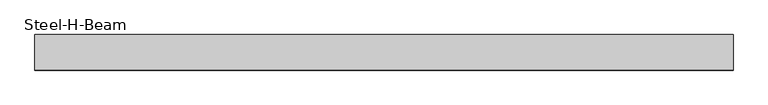
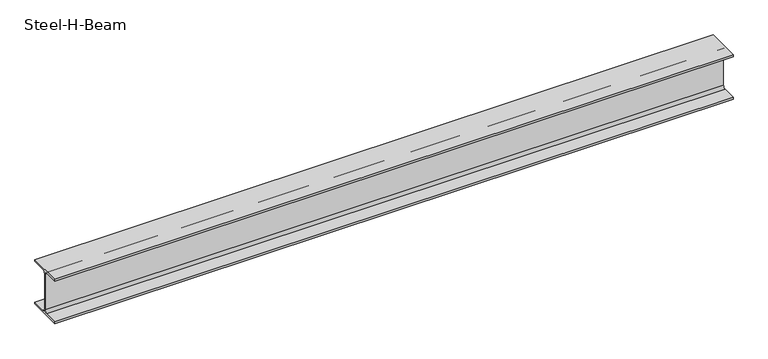
"""IFC4 building model written with IfcOpenShell, lengths in millimetres: beam geometry, Steel-H-Beam : BM121_H-340×250x9x14."""

from ifc_helpers import new_model, si_unit, point, frame, frame_2d, origin, place, context, project, spatial, polyline, circle_curve, trimmed, segment, composite_curve, outline, extrude, source, transform, mapped, element, save


def steel_h_beam_5215ea41(model_context):
    return source(origin(), model_context, "Body", "SweptSolid", [
        extrude(outline(composite_curve([segment(polyline([(-125.0, -156.0), (-24.5, -156.0)]), True, "CONTINUOUS"), segment(trimmed(circle_curve(frame_2d((-24.5, -136.0)), 20.0), [point((-24.5, -156.0))], [point((-4.5, -136.0))], True, "CARTESIAN"), True, "CONTINUOUS"), segment(polyline([(-4.5, -136.0), (-4.5, 136.0)]), True, "CONTINUOUS"), segment(trimmed(circle_curve(frame_2d((-24.5, 136.0)), 20.0), [point((-4.5, 136.0))], [point((-24.5, 156.0))], True, "CARTESIAN"), True, "CONTINUOUS"), segment(polyline([(-24.5, 156.0), (-125.0, 156.0), (-125.0, 170.0), (125.0, 170.0), (125.0, 156.0), (24.5, 156.0)]), True, "CONTINUOUS"), segment(trimmed(circle_curve(frame_2d((24.5, 136.0)), 20.0), [point((24.5, 156.0))], [point((4.5, 136.0))], True, "CARTESIAN"), True, "CONTINUOUS"), segment(polyline([(4.5, 136.0), (4.5, -136.0)]), True, "CONTINUOUS"), segment(trimmed(circle_curve(frame_2d((24.5, -136.0)), 20.0), [point((4.5, -136.0))], [point((24.5, -156.0))], True, "CARTESIAN"), True, "CONTINUOUS"), segment(polyline([(24.5, -156.0), (125.0, -156.0), (125.0, -170.0), (-125.0, -170.0), (-125.0, -156.0)]), True, "CONTINUOUS")], self_intersect=False)), frame((-2363.9803034, 0.0, 0.0), z_axis=(1.0, 0.0, 0.0), x_axis=(0.0, 1.0, 0.0)), (0.0, 0.0, 1.0), 4905.0160952),
    ])


if __name__ == "__main__":
    model = new_model("IFC4")
    model_context = context("Model", 3, world=origin())
    ifc_project = project(units=[si_unit("LENGTHUNIT", "METRE", prefix="MILLI")], contexts=[model_context])
    site = spatial("IfcSite", under=ifc_project)
    building = spatial("IfcBuilding", under=site)
    placement = place(None, origin())
    steel_h_beam_shape = steel_h_beam_5215ea41(model_context)
    element("IfcBeam", 1, ObjectType="Steel-H-Beam : BM121_H-340×250x9x14", at=placement, inside=building, context=model_context, shape_type="MappedRepresentation", body=[
        mapped(steel_h_beam_shape, transform((0.0, 0.0, 0.0), x_axis=(1.0, 0.0, 0.0), y_axis=(0.0, 1.0, 0.0), z_axis=(0.0, 0.0, 1.0))),
    ])
    save(model, "model.ifc")

# Revit data of these elements
# Type "Steel-H-Beam : BM121_H-340×250x9x14"
#   Surface Area = 1.62766 m²/m
#   Section Area = 101.514 cm²
#   Mass per Unit Length = 79.6882 kg/m
#   Length [instance default] = 3000 mm
#   B = 250 mm
#   H = 340 mm
#   r = 20 mm
#   tw = 9 mm
#   tf = 14 mm
#   hec_material4 [instance default] = none
#   hec_material3 [instance default] = none
#   hec_material2 [instance default] = none
#   hec_material1 [instance default] = none
#   Structural Material [instance default] = Steel, 45-345
#   Assembly Code = ""
# Element 1 (IfcBeam, "Steel-H-Beam : BM121_H-340×250x9x14")
#   hec_material4 = S01AA010-00002_Main Steel Structure Fabrication Work_Shelter/Building_Steel Painting/Coating_for Fireproofed Steel Surface, Surface Preparation & Primer Coat
#   hec_material3 = F01AC000-00002_Building/Shelter Fire Proofing Work_Intumescent Coating Type_1 hr. rating (UL 1709))
#   hec_material2 = S01AA010-00002_Main Steel Structure Fabrication Work_Shelter/Building_Steel Painting/Coating_for Fireproofed Steel Surface, Surface Preparation & Primer Coat
#   hec_material1 = S03AA028-00001_Main Steel Structure Erection Work_Shelter/Building_Medium Steel
#   Structural Material = S01AA002-00001_Main Steel Structure Fabrication Work_Shelter/Building_Medium Steel - Standard
#   Materials on its faces: "S01AA002-00001_Main Steel Structure Fabrication Work_Shelter/Building_Medium Steel - Standard"
# Materials
#   "Steel, 45-345": class "Metal", colour RGB 189 187 185, transparency 0, Description = "Steel 345 MPa", Cost = 0
#   "S01AA002-00001_Main Steel Structure Fabrication Work_Shelter/Building_Medium Steel - Standard": class "Metal", colour RGB 120 120 120, transparency 0, Comments = "(90KG/M>Weight≥30KG/M)", Description = "Structural steel 50ksi", W00) Work Master Code = "S01AA002-0001", W01) Work Master_Lv1 = "Main Steel Structure Fabrication Work", W02) Work Master_Lv2 = "Shelter/Building", W03) Work Master_Spec.1 = "Medium Steel - Standard (90KG/M>Weight≥30KG/M)", Cost = 0
#   "S01AA010-00002_Main Steel Structure Fabrication Work_Shelter/Building_Steel Painting/Coating_for Fireproofed Steel Surface, Surface Preparation & Primer Coat": class "Metal", colour RGB 120 120 120, transparency 0, Description = "Paint finished steel", W00) Work Master Code = "SS01AA010-00002", W01) Work Master_Lv1 = "Main Steel Structure Fabrication Work", W02) Work Master_Lv2 = "Shelter/Building", W03) Work Master_Spec.1 = "Steel Painting/Coating", W04) Work Master_Spec.2 = "for Fireproofed Steel Surface, Surface Preparation & Primer Coat", Cost = 0
#   "F01AC000-00002_Building/Shelter Fire Proofing Work_Intumescent Coating Type_1 hr. rating (UL 1709))": class "Metal", colour RGB 255 128 128, transparency 0, Description = "Paint finished steel", W00) Work Master Code = "F01AC000-00002", W01) Work Master_Lv1 = "Building/Shelter Fire Proofing Work", W02) Work Master_Lv2 = "Intumescent Coating Type", W03) Work Master_Spec.1 = "1 hr. rating (UL 1709)", Cost = 0
#   "S03AA028-00001_Main Steel Structure Erection Work_Shelter/Building_Medium Steel": class "Metal", colour RGB 120 120 120, transparency 0, Comments = "(90KG/M>Weight≥30KG/M)", Description = "Structural steel 50ksi", W00) Work Master Code = "S03AA028-0001", W01) Work Master_Lv1 = "Main Steel Structure Erection Work", W02) Work Master_Lv2 = "Shelter/Building", W03) Work Master_Spec.1 = "Medium Steel (90KG/M>Weight≥30KG/M)", Cost = 0
